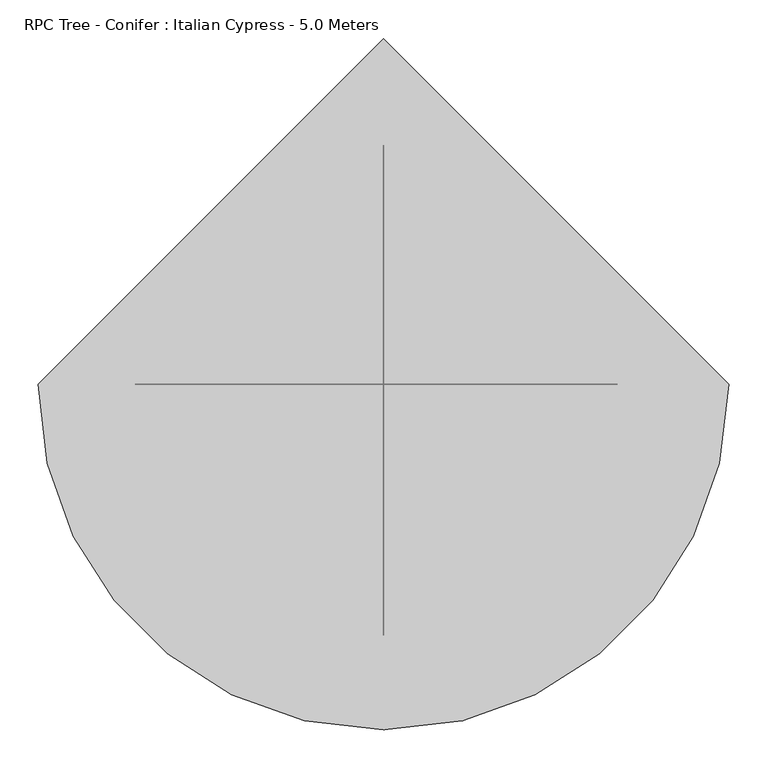
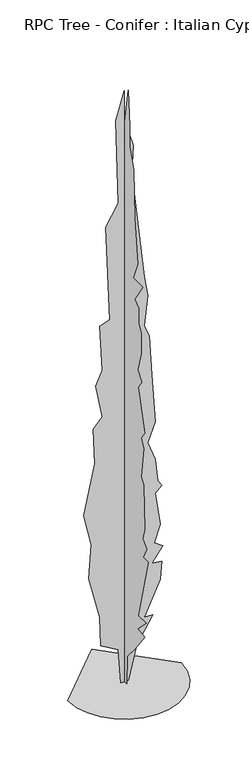
"""IFC4 building model written with IfcOpenShell, lengths in millimetres: geographic element geometry, RPC Tree - Conifer : Italian Cypress - 5.0 Meters."""

import ifcopenshell
import ifcopenshell.guid

model = None  # the IFC model being written
_history = None  # IfcOwnerHistory: only IFC2X3 demands one
_inside = {}  # id of a spatial element -> (the spatial element, [elements in it])
_under = {}  # id of a project, library or spatial element -> (it, [spatial elements below it])
_declared = {}  # id of a project -> (the project, [libraries it declares])
_typed = {}  # id of a type object -> (the type object, [elements of that type])
_made_of = {}  # id of a material, layer set ... -> (it, [elements and type objects made of it])


def new_model(schema):
    """Start an empty IFC model of exactly this schema.

    Asked for "IFC4X3", IfcOpenShell would pick the latest addendum, in which some entities
    have other attributes; the version numbers below select the first issue.
    IFC2X3 requires an IfcOwnerHistory on every rooted entity: one is made here for all.
    """
    global model, _history
    if schema == "IFC4X3":
        model = ifcopenshell.file(schema_version=(4, 3, 0, 0))
    else:
        model = ifcopenshell.file(schema=schema)
    _inside.clear()
    _under.clear()
    _declared.clear()
    _typed.clear()
    _made_of.clear()
    _history = None
    if model.schema == "IFC2X3":
        org = make("IfcOrganization", Name="unknown")
        user = make(
            "IfcPersonAndOrganization",
            ThePerson=make("IfcPerson", FamilyName="unknown"),
            TheOrganization=org,
        )
        app = make(
            "IfcApplication",
            ApplicationDeveloper=org,
            Version="unknown",
            ApplicationFullName="unknown",
            ApplicationIdentifier="unknown",
        )
        _history = make(
            "IfcOwnerHistory",
            OwningUser=user,
            OwningApplication=app,
            ChangeAction="ADDED",
            CreationDate=0,
        )
    return model


def make(cls, **values):
    """One entity of the class cls with the attributes given. An attribute that is None is left unset."""
    return model.create_entity(
        cls, **{name: value for name, value in values.items() if value is not None}
    )


def rooted(cls, **values):
    """An entity with a GlobalId (a new one), such as an element, a storey or a relation."""
    return make(cls, GlobalId=ifcopenshell.guid.new(), OwnerHistory=_history, **values)


def si_unit(unit_type, name, prefix=None):
    """IfcSIUnit, for example si_unit("LENGTHUNIT", "METRE", prefix="MILLI")."""
    return make("IfcSIUnit", UnitType=unit_type, Prefix=prefix, Name=name)


def assignment(units):
    """IfcUnitAssignment: the units of a project."""
    return None if units is None else make("IfcUnitAssignment", Units=units)


def point(xyz):
    """IfcCartesianPoint."""
    return None if xyz is None else make("IfcCartesianPoint", Coordinates=xyz)


def direction(xyz):
    """IfcDirection."""
    return None if xyz is None else make("IfcDirection", DirectionRatios=xyz)


def frame(location, z_axis=None, x_axis=None):
    """IfcAxis2Placement3D, a coordinate frame: its origin and axes. An axis left out is left unset."""
    return make(
        "IfcAxis2Placement3D",
        Location=point(location),
        Axis=direction(z_axis),
        RefDirection=direction(x_axis),
    )


def origin():
    """The frame at (0, 0, 0) with its axes left unset."""
    return frame((0.0, 0.0, 0.0))


def place(relative_to, where):
    """IfcLocalPlacement: puts the frame where relative to a parent placement (None: the world)."""
    return make(
        "IfcLocalPlacement", PlacementRelTo=relative_to, RelativePlacement=where
    )


def context(
    kind, dimensions, precision=None, world=None, true_north=None, identifier=None
):
    """IfcGeometricRepresentationContext, for example the 3D "Model" context."""
    return make(
        "IfcGeometricRepresentationContext",
        ContextIdentifier=identifier,
        ContextType=kind,
        CoordinateSpaceDimension=dimensions,
        Precision=precision,
        WorldCoordinateSystem=world,
        TrueNorth=true_north,
    )


def project(units=None, contexts=None):
    """IfcProject with its units and contexts."""
    return rooted(
        "IfcProject",
        Name="project",
        RepresentationContexts=contexts,
        UnitsInContext=assignment(units),
    )


def spatial(cls, under=None, at=None, **own):
    """A site, building, storey or space (cls), placed at a placement, below another one or the project."""
    s = rooted(cls, ObjectPlacement=at, **own)
    if under is not None:
        _under.setdefault(under.id(), (under, []))[1].append(s)
    return s


def point_list(points):
    """IfcCartesianPointList2D or 3D."""
    cls = (
        "IfcCartesianPointList2D" if len(points[0]) == 2 else "IfcCartesianPointList3D"
    )
    return make(cls, CoordList=points)


def triangles(points, corners, closed=None, point_numbers=None):
    """IfcTriangulatedFaceSet: each triangle names its three corners, points numbered from 1."""
    return make(
        "IfcTriangulatedFaceSet",
        Coordinates=point_list(points),
        Closed=closed,
        CoordIndex=corners,
        PnIndex=point_numbers,
    )


def shape(context_of_items, identifier, shape_type, items):
    """IfcShapeRepresentation: the items that make up one representation, for example the "Body"."""
    return make(
        "IfcShapeRepresentation",
        ContextOfItems=context_of_items,
        RepresentationIdentifier=identifier,
        RepresentationType=shape_type,
        Items=items,
    )


def source(mapping_origin, context_of_items, identifier, shape_type, items):
    """IfcRepresentationMap: a shape defined once, which mapped items show again and again."""
    return make(
        "IfcRepresentationMap",
        MappingOrigin=mapping_origin,
        MappedRepresentation=shape(context_of_items, identifier, shape_type, items),
    )


def transform(
    local_origin,
    x_axis=None,
    y_axis=None,
    z_axis=None,
    scale=None,
    scale2=None,
    scale3=None,
    uniform=True,
):
    """IfcCartesianTransformationOperator3D, or its non-uniform kind. x_axis, y_axis, z_axis: its Axis1, 2, 3."""
    if uniform:
        return make(
            "IfcCartesianTransformationOperator3D",
            Axis1=direction(x_axis),
            Axis2=direction(y_axis),
            LocalOrigin=point(local_origin),
            Scale=scale,
            Axis3=direction(z_axis),
        )
    return make(
        "IfcCartesianTransformationOperator3DnonUniform",
        Axis1=direction(x_axis),
        Axis2=direction(y_axis),
        LocalOrigin=point(local_origin),
        Scale=scale,
        Axis3=direction(z_axis),
        Scale2=scale2,
        Scale3=scale3,
    )


def mapped(mapping_source, mapping_target):
    """IfcMappedItem: shows the shape of a source again, moved by a transform."""
    return make(
        "IfcMappedItem", MappingSource=mapping_source, MappingTarget=mapping_target
    )


def made_of(thing, what):
    """Note that an element or type object is made of a material, layer set ...; save() writes the relation."""
    if what is not None:
        _made_of.setdefault(what.id(), (what, []))[1].append(thing)
    return thing


def element(
    cls,
    number,
    at=None,
    inside=None,
    cuts=None,
    type_object=None,
    material=None,
    context=None,
    identifier="Body",
    shape_type=None,
    held_by="IfcProductDefinitionShape",
    body=None,
    shapes=None,
    **own,
):
    """One element of the class cls, such as IfcWall. Its Tag is "e" and its number.

    at: its placement. inside: the storey or other place that contains it. cuts: it is an
    opening in that element (IfcRelVoidsElement). A single representation is given by context,
    identifier, shape_type and body (its items); several are given by shapes. held_by: the class
    of the entity that holds the representations. save() writes the other relations.
    """
    e = rooted(cls, Tag="e%d" % number, ObjectPlacement=at, **own)
    if body is not None:
        shapes = [shape(context, identifier, shape_type, body)]
    if shapes is not None:
        e.Representation = make(held_by, Representations=shapes)
    if inside is not None:
        _inside.setdefault(inside.id(), (inside, []))[1].append(e)
    if cuts is not None:
        rooted(
            "IfcRelVoidsElement", RelatingBuildingElement=cuts, RelatedOpeningElement=e
        )
    if type_object is not None:
        _typed.setdefault(type_object.id(), (type_object, []))[1].append(e)
    return made_of(e, material)


def aggregate(whole, parts):
    """IfcRelAggregates: a whole, such as a stair, and the parts it consists of."""
    return rooted("IfcRelAggregates", RelatingObject=whole, RelatedObjects=parts)


def save(model, path):
    """Write the relations noted so far, then the file.

    IfcRelAggregates (storeys below a building ...), IfcRelContainedInSpatialStructure (elements
    in a storey), IfcRelDefinesByType, IfcRelAssociatesMaterial and IfcRelDeclares: one each for
    every whole, place, type object, material and project.
    """
    for whole, parts in _under.values():
        aggregate(whole, parts)
    for where, things in _inside.values():
        rooted(
            "IfcRelContainedInSpatialStructure",
            RelatedElements=things,
            RelatingStructure=where,
        )
    for kind, things in _typed.values():
        rooted("IfcRelDefinesByType", RelatedObjects=things, RelatingType=kind)
    for what, things in _made_of.values():
        rooted("IfcRelAssociatesMaterial", RelatedObjects=things, RelatingMaterial=what)
    for by, libraries in _declared.values():
        rooted("IfcRelDeclares", RelatingContext=by, RelatedDefinitions=libraries)
    model.write(path)


def rpc_tree_conifer_italian_cypress_5_0_meters_3d53936f(model_context):
    return source(origin(), model_context, "Body", "Tessellation", [
        triangles([(-28.9243291, 1.3e-06, 0.1175505), (-48.5995771, -1.5e-05, 287.7924989), (-186.3258362, -1.37e-05, 366.4949987), (-196.1633353, -2.79e-05, 612.4350014), (-284.7008453, -4.52e-05, 966.5875122), (-265.0258289, -6.24e-05, 1242.0400303), (-324.0508235, -7.57e-05, 1507.6550674), (-235.513586, -0.0001036, 1910.9949829), (-245.3513394, -0.0001208, 2206.1249336), (-176.4880827, -0.0001285, 2284.8250717), (-225.6760869, -0.0001427, 2560.275119), (-176.4880827, -0.0001519, 2678.3248901), (-196.1633353, -0.0001733, 3052.1500374), (-117.4625795, -0.0001785, 3081.6749794), (-146.9753311, -0.0002242, 3868.6749069), (-48.5993273, -0.0002384, 4035.9248726), (-68.2745799, -0.0002792, 4734.3749725), (0.5886036, -0.0002957, 4960.6501144), (0.5885936, -0.0002816, 4724.5499908), (69.4516701, -0.00027, 4478.5998871), (59.614171, -0.0002561, 4252.3500343), (157.9899204, -0.0002064, 3347.2750465), (187.5026721, -0.0001977, 3180.0500793), (157.9899204, -0.0001818, 2934.0999756), (197.3401711, -0.0001776, 2835.7248756), (217.0154055, -0.0001586, 2501.2499428), (246.5281571, -0.0001358, 2097.9100273), (187.5026721, -0.0001239, 1940.5100418), (246.5281571, -0.000117, 1783.1074402), (266.2041545, -0.0001068, 1596.1925411), (295.71667, -0.0001051, 1547.0049911), (246.5281571, -0.0001, 1497.8174412), (285.8791709, -8.53e-05, 1222.3650684), (236.690658, -7.5e-05, 1084.6375013), (305.5541691, -7.51e-05, 1035.450024), (217.0154055, -6.42e-05, 917.4000349), (295.71667, -6.7e-05, 907.5624813), (285.8791709, -5.78e-05, 759.997506), (157.9899204, -3.58e-05, 484.5449879), (226.8529046, -3.88e-05, 484.5449879), (98.9641719, -2.09e-05, 277.9549998), (30.1011696, -1.3e-06, 0.058986), (0.1966738, 26.4907499, 3.55e-05), (0.1966807, 16.6530749, 238.6054939), (0.196685, 95.3537455, 258.2800016), (0.196697, 203.5672438, 494.3825051), (0.1967129, 311.7799882, 819.0224642), (0.1967124, 233.0799954, 887.8875195), (0.1967188, 242.9174945, 1094.4749823), (0.1967282, 272.4299918, 1419.1174484), (0.1967333, 262.5924927, 1547.0049911), (0.1967324, 213.4047429, 1645.3799458), (0.1967414, 272.4299918, 1861.8074329), (0.1967478, 193.7295085, 2156.9350582), (0.196749, 174.0544922, 2274.9874454), (0.1967577, 223.242242, 2422.54995), (0.1967593, 164.2167569, 2658.6499283), (0.1967653, 174.054256, 2786.5499702), (0.1967665, 134.7039962, 2924.2749939), (0.1967759, 154.3792578, 3189.875061), (0.1967755, 85.5160011, 3317.775103), (0.1967853, 124.8664971, 3504.675032), (0.19679, 75.678502, 3799.8250397), (0.1967981, 36.3279992, 4094.9500488), (0.1968071, 65.8407486, 4340.8748634), (0.1968079, 26.4905001, 4468.7749054), (0.1968139, -3.0223, 4704.875029), (0.1968216, -52.2102488, 5000.0000381), (0.1968108, -71.8855014, 4704.875029), (0.1968066, -71.8855014, 4537.6250633), (0.1968002, -130.9109955, 4380.2250778), (0.1967852, -140.7485037, 3976.899987), (0.1967737, -180.0987453, 3612.9001122), (0.1967729, -121.0732512, 3465.3251083), (0.1967673, -248.962002, 3465.3251083), (0.1967647, -140.7485037, 3298.1001411), (0.1967635, -199.7739979, 3258.7499268), (0.1967579, -199.7739979, 3130.8498848), (0.1967536, -229.2867495, 3062.0000175), (0.1967493, -229.2867495, 2894.7500519), (0.1967472, -180.0987453, 2727.5250847), (0.1967416, -239.1242486, 2658.6499283), (0.1967438, -189.9364988, 2589.800061), (0.1967284, -278.475008, 2255.3124836), (0.1967275, -229.2867495, 2186.4499718), (0.1967259, -268.6375089, 2117.5849892), (0.1967195, -229.2867495, 1861.8074329), (0.1967156, -268.6375089, 1812.6200283), (0.1967054, -278.475008, 1448.6300365), (0.1967024, -248.9617477, 1350.2524658), (0.1966976, -307.9874871, 1301.0650612), (0.1966986, -258.7999917, 1202.6900339), (0.1966956, -327.6624853, 1202.6900339), (0.1966845, -189.9362444, 671.4600323), (0.1966797, -298.1500062, 671.4600323), (0.1966828, -180.0987453, 553.4074997), (0.1966781, -278.475008, 543.5699824), (0.196679, -150.5860028, 366.4949987), (0.1966781, -42.3724999, 238.6054939), (0.1966712, -32.534751, 3.2e-05), (-450.413314, 0.0, 5.36e-05), (-438.5008143, -103.2502475, 4.7e-05), (-404.5758139, -198.0692509, 3.98e-05), (-351.3483215, -281.7399977, 3.25e-05), (-281.5433345, -351.54751, 2.53e-05), (-197.8723334, -404.7699881, 1.85e-05), (-103.0535753, -438.6974957, 1.23e-05), (0.1966927, -450.6125024, 7.1e-06), (103.4469197, -438.6974957, 3.3e-06), (198.2659141, -404.7724952, 1.1e-06), (281.9366608, -351.5450028, 7e-07), (351.7441913, -281.7399977, 1.8e-06), (404.9666694, -198.0689966, 4.4e-06), (438.894177, -103.2502475, 8.6e-06), (450.8066766, 3.94e-05, 1.42e-05), (0.1966127, 450.6125024, 6.08e-05)], [[17, 18, 19], [39, 40, 41], [16, 17, 19], [16, 19, 20], [16, 20, 21], [16, 21, 22], [15, 16, 22], [14, 15, 22], [14, 22, 23], [14, 23, 24], [34, 35, 36], [36, 37, 38], [42, 1, 2], [41, 42, 2], [39, 41, 2], [30, 31, 32], [39, 2, 3], [39, 3, 4], [38, 39, 4], [36, 38, 4], [36, 4, 5], [34, 36, 5], [34, 5, 6], [33, 34, 6], [32, 33, 6], [32, 6, 7], [32, 7, 8], [30, 32, 8], [29, 30, 8], [28, 29, 8], [28, 8, 9], [27, 28, 9], [27, 9, 10], [26, 27, 10], [26, 10, 11], [26, 11, 12], [25, 26, 12], [25, 12, 13], [24, 25, 13], [14, 24, 13], [67, 68, 69], [94, 95, 96], [74, 75, 76], [96, 97, 98], [92, 93, 94], [100, 43, 44], [99, 100, 44], [67, 69, 70], [66, 67, 70], [66, 70, 71], [65, 66, 71], [65, 71, 72], [64, 65, 72], [63, 64, 72], [63, 72, 73], [62, 63, 73], [62, 73, 74], [61, 62, 74], [61, 74, 76], [90, 91, 92], [81, 82, 83], [46, 47, 48], [60, 61, 76], [59, 60, 76], [59, 76, 77], [59, 77, 78], [59, 78, 79], [59, 79, 80], [59, 80, 81], [58, 59, 81], [57, 58, 81], [57, 81, 83], [56, 57, 83], [56, 83, 84], [55, 56, 84], [55, 84, 85], [54, 55, 85], [53, 54, 85], [53, 85, 86], [53, 86, 87], [52, 53, 87], [52, 87, 88], [52, 88, 89], [51, 52, 89], [51, 89, 90], [50, 51, 90], [49, 50, 90], [49, 90, 92], [49, 92, 94], [48, 49, 94], [46, 48, 94], [46, 94, 96], [46, 96, 98], [45, 46, 98], [45, 98, 99], [44, 45, 99], [115, 116, 101], [114, 115, 101], [114, 101, 102], [113, 114, 102], [113, 102, 103], [113, 103, 104], [112, 113, 104], [111, 112, 104], [111, 104, 105], [111, 105, 106], [111, 106, 107], [111, 107, 108], [111, 108, 109], [111, 109, 110]], closed=False),
    ])


if __name__ == "__main__":
    model = new_model("IFC4")
    model_context = context("Model", 3, world=origin())
    ifc_project = project(units=[si_unit("LENGTHUNIT", "METRE", prefix="MILLI")], contexts=[model_context])
    site = spatial("IfcSite", under=ifc_project)
    building = spatial("IfcBuilding", under=site)
    placement = place(None, origin())
    rpc_tree_conifer_italian_cypress_5_0_meters_shape = rpc_tree_conifer_italian_cypress_5_0_meters_3d53936f(model_context)
    element("IfcGeographicElement", 1, ObjectType="RPC Tree - Conifer : Italian Cypress - 5.0 Meters", at=placement, inside=building, context=model_context, shape_type="MappedRepresentation", body=[
        mapped(rpc_tree_conifer_italian_cypress_5_0_meters_shape, transform((0.0, 0.0, 0.0), x_axis=(1.0, 0.0, 0.0), y_axis=(0.0, 1.0, 0.0), z_axis=(0.0, 0.0, 1.0))),
    ])
    save(model, "model.ifc")

# Revit data of these elements
# Project information
#   Document_Suitability_Code = "A1"
#   Document_Suitability_Description = "Coordination"
#   Project Status = "Project Status"
#   Client Name = "Revit Project"
#   Project Address = "Limerick Institute of Technology"
#   Project Name = "Commercial Units"
#   Project Number = "RARC02"
# Type "RPC Tree - Conifer : Italian Cypress - 5.0 Meters"
#   built-in parameter 1005198 = "{2, 15},{39, RPC-16-FWM7-6P00-C8X0-C000-ST1L-LVER-AU},{1, 0},{1, 0},{2, 13},{1, 8},{5, Color},{1, 0},{1, 0},{3, 0.8},{3, 0.8},{3, 0.8},{1, 8},{7, BBoxMin},{1, 0},{1, 0},{1, 0},{1, 0},{1, 0},{1, 8},{7, BBoxMax},{1, 0},{1, 0},{1, 0},{1, 0},{1, 0},{2, 11},{9, RPCTypeId},{1, 0},{1, 0},{39, RPC-16-FWM7-6P00-C8X0-C000-ST1L-LVER-AU},{1, 6},{14, RPCPlantHeight},{1, 0},{1, 0},{7, 16.4042},{2, 11},{7, keyword},{1, 0},{1, 0},{34, :RPCs:Trees [General]:Geometry:RPC},{2, 11},{8, category},{1, 0},{1, 0},{15, Trees [General]},{2, 11},{12, LocalizedUID},{1, 0},{1, 0},{15, Italian Cypress},{2, 14},{6, Height},{1, 0},{1, 0},{7, 16.4042},{1, 2},{16, Cast Reflections},{1, 0},{1, 0},{1, 0},{1, 2},{12, Cast Shadows},{1, 0},{1, 0},{1, 1},{1, 2},{9, Lock View},{1, 0},{1, 0},{1, 0},{1, 4},{5, ViewC},{1, 0},{1, 0},{1, 0},{21, assetlibrary_base.fbx},{1, 5},"
#   built-in parameter 1005195 = "RPC-16-FWM7-6P00-C8X0-C000-ST1L-LVER-AU"
#   Type Comments = "Italian Cypress"
#   Height = 5000 mm
#   Description = (empty or 0)
#   Default Elevation = 0
